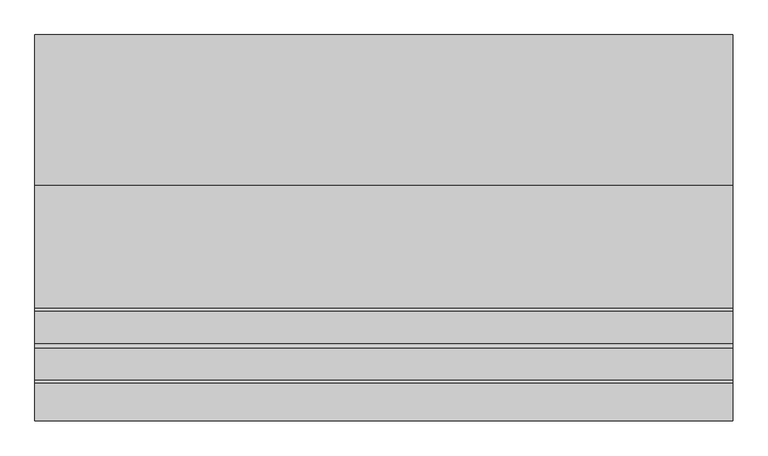
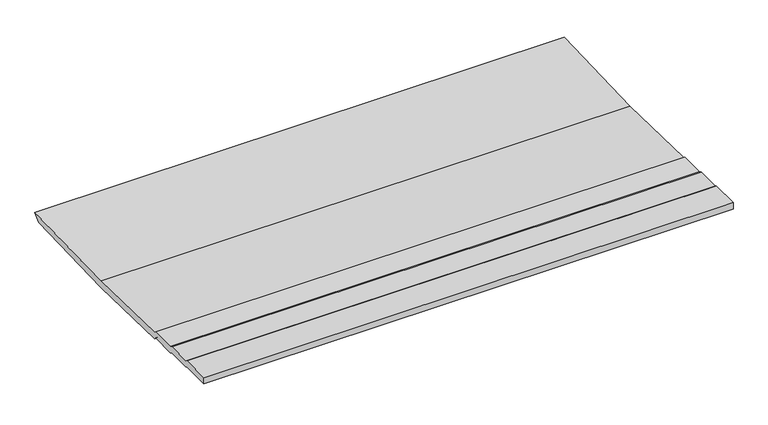
"""IFC4 building model written with IfcOpenShell, lengths in millimetres: proxy geometry, GRAVEL BALLAST1:GRAVEL BALLAST002:288722 : GRAVEL BALLAST1:GRAVEL BALLAST002:288722."""

from ifc_helpers import new_model, si_unit, frame, origin, place, context, project, spatial, polyline, outline, extrude, source, transform, mapped, element, save


def generic_models_dad5ae01(model_context):
    return source(origin(), model_context, "Body", "SweptSolid", [
        extrude(outline(polyline([(-5153.3229276, 40249.5125), (-5162.0333769, 40253.79375), (-5271.5328886, 40253.79375), (-5271.5328886, 40278.5320313), (-5162.0333769, 40278.5320313), (-5153.3229276, 40274.2507813), (-5062.7360136, 40274.2507813), (-5049.8913742, 40268.5233193), (-4955.9396269, 40270.16875), (-4947.6661894, 40262.7585938), (-4595.1095487, 40254.5398438), (-4164.5068144, 40268.1982422), (-4189.7324003, 40242.9726562), (-4595.1095487, 40229.8015625), (-4947.6661894, 40238.0203125), (-4955.9396269, 40245.4304687), (-5049.8913742, 40243.785038), (-5062.7360136, 40249.5125), (-5153.3229276, 40249.5125)])), frame((17159.7769925, 0.0, 0.0), z_axis=(1.0, 0.0, 0.0), x_axis=(0.0, 1.0, 0.0)), (0.0, 0.0, 1.0), 2000.0),
    ])


if __name__ == "__main__":
    model = new_model("IFC4")
    model_context = context("Model", 3, world=origin())
    ifc_project = project(units=[si_unit("LENGTHUNIT", "METRE", prefix="MILLI")], contexts=[model_context])
    site = spatial("IfcSite", under=ifc_project)
    building = spatial("IfcBuilding", under=site)
    placement = place(None, origin())
    generic_models_shape = generic_models_dad5ae01(model_context)
    element("IfcBuildingElementProxy", 1, Name="GRAVEL BALLAST1:GRAVEL BALLAST002:288722 : GRAVEL BALLAST1:GRAVEL BALLAST002:288722", ObjectType="GRAVEL BALLAST1:GRAVEL BALLAST002:288722 : GRAVEL BALLAST1:GRAVEL BALLAST002:288722", at=placement, inside=building, context=model_context, shape_type="MappedRepresentation", body=[
        mapped(generic_models_shape, transform((0.0, 0.0, 0.0), x_axis=(1.0, 0.0, 0.0), y_axis=(0.0, 1.0, 0.0), z_axis=(0.0, 0.0, 1.0))),
    ])
    save(model, "model.ifc")

# Revit data of these elements
# Type "GRAVEL BALLAST1:GRAVEL BALLAST002:288722 : GRAVEL BALLAST1:GRAVEL BALLAST002:288722"
#   NameOverride = "GRAVEL BALLAST1:GRAVEL BALLAST002:288722"
#   ObjectTypeOverride = "GRAVEL BALLAST1:GRAVEL BALLAST002"
#   Reference = "GRAVEL BALLAST002"
#   Category = "Generic Models"
#   Tag = "288722"
# Element 1 (IfcBuildingElementProxy, "GRAVEL BALLAST1:GRAVEL BALLAST002:288722 : GRAVEL BALLAST1:GRAVEL BALLAST002:288722")
#   Materials on its faces: "GRAVEL BALLAST"
# Materials
#   "GRAVEL BALLAST": class "Unassigned", colour RGB 128 128 128, transparency 0, Cost = 0
